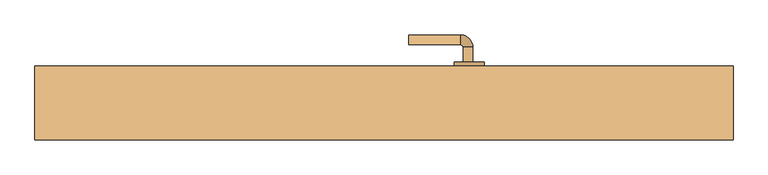
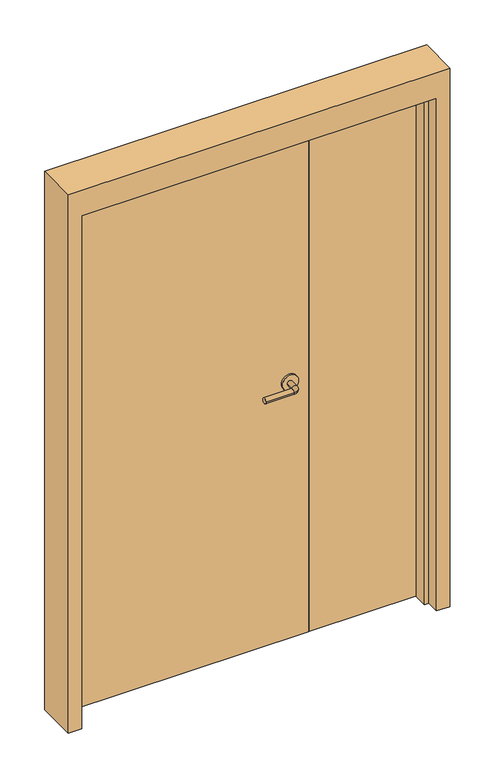
"""IFC4 building model written with IfcOpenShell, lengths in millimetres: door geometry, Дверь-Маятниковая-С полотнами разной ширины-Щитовая : 1410 x 2100 мм."""

import ifcopenshell
import ifcopenshell.guid

model = None  # the IFC model being written
_history = None  # IfcOwnerHistory: only IFC2X3 demands one
_inside = {}  # id of a spatial element -> (the spatial element, [elements in it])
_under = {}  # id of a project, library or spatial element -> (it, [spatial elements below it])
_declared = {}  # id of a project -> (the project, [libraries it declares])
_typed = {}  # id of a type object -> (the type object, [elements of that type])
_made_of = {}  # id of a material, layer set ... -> (it, [elements and type objects made of it])


def new_model(schema):
    """Start an empty IFC model of exactly this schema.

    Asked for "IFC4X3", IfcOpenShell would pick the latest addendum, in which some entities
    have other attributes; the version numbers below select the first issue.
    IFC2X3 requires an IfcOwnerHistory on every rooted entity: one is made here for all.
    """
    global model, _history
    if schema == "IFC4X3":
        model = ifcopenshell.file(schema_version=(4, 3, 0, 0))
    else:
        model = ifcopenshell.file(schema=schema)
    _inside.clear()
    _under.clear()
    _declared.clear()
    _typed.clear()
    _made_of.clear()
    _history = None
    if model.schema == "IFC2X3":
        org = make("IfcOrganization", Name="unknown")
        user = make(
            "IfcPersonAndOrganization",
            ThePerson=make("IfcPerson", FamilyName="unknown"),
            TheOrganization=org,
        )
        app = make(
            "IfcApplication",
            ApplicationDeveloper=org,
            Version="unknown",
            ApplicationFullName="unknown",
            ApplicationIdentifier="unknown",
        )
        _history = make(
            "IfcOwnerHistory",
            OwningUser=user,
            OwningApplication=app,
            ChangeAction="ADDED",
            CreationDate=0,
        )
    return model


def make(cls, **values):
    """One entity of the class cls with the attributes given. An attribute that is None is left unset."""
    return model.create_entity(
        cls, **{name: value for name, value in values.items() if value is not None}
    )


def rooted(cls, **values):
    """An entity with a GlobalId (a new one), such as an element, a storey or a relation."""
    return make(cls, GlobalId=ifcopenshell.guid.new(), OwnerHistory=_history, **values)


def si_unit(unit_type, name, prefix=None):
    """IfcSIUnit, for example si_unit("LENGTHUNIT", "METRE", prefix="MILLI")."""
    return make("IfcSIUnit", UnitType=unit_type, Prefix=prefix, Name=name)


def assignment(units):
    """IfcUnitAssignment: the units of a project."""
    return None if units is None else make("IfcUnitAssignment", Units=units)


def point(xyz):
    """IfcCartesianPoint."""
    return None if xyz is None else make("IfcCartesianPoint", Coordinates=xyz)


def direction(xyz):
    """IfcDirection."""
    return None if xyz is None else make("IfcDirection", DirectionRatios=xyz)


def frame(location, z_axis=None, x_axis=None):
    """IfcAxis2Placement3D, a coordinate frame: its origin and axes. An axis left out is left unset."""
    return make(
        "IfcAxis2Placement3D",
        Location=point(location),
        Axis=direction(z_axis),
        RefDirection=direction(x_axis),
    )


def frame_2d(location, x_axis=None):
    """IfcAxis2Placement2D, a coordinate frame in the plane: its origin and x axis."""
    return make(
        "IfcAxis2Placement2D", Location=point(location), RefDirection=direction(x_axis)
    )


def origin():
    """The frame at (0, 0, 0) with its axes left unset."""
    return frame((0.0, 0.0, 0.0))


def origin_with_axes():
    """The frame at (0, 0, 0) with the z axis (0, 0, 1) and the x axis (1, 0, 0) written out."""
    return frame((0.0, 0.0, 0.0), z_axis=(0.0, 0.0, 1.0), x_axis=(1.0, 0.0, 0.0))


def place(relative_to, where):
    """IfcLocalPlacement: puts the frame where relative to a parent placement (None: the world)."""
    return make(
        "IfcLocalPlacement", PlacementRelTo=relative_to, RelativePlacement=where
    )


def context(
    kind, dimensions, precision=None, world=None, true_north=None, identifier=None
):
    """IfcGeometricRepresentationContext, for example the 3D "Model" context."""
    return make(
        "IfcGeometricRepresentationContext",
        ContextIdentifier=identifier,
        ContextType=kind,
        CoordinateSpaceDimension=dimensions,
        Precision=precision,
        WorldCoordinateSystem=world,
        TrueNorth=true_north,
    )


def project(units=None, contexts=None):
    """IfcProject with its units and contexts."""
    return rooted(
        "IfcProject",
        Name="project",
        RepresentationContexts=contexts,
        UnitsInContext=assignment(units),
    )


def spatial(cls, under=None, at=None, **own):
    """A site, building, storey or space (cls), placed at a placement, below another one or the project."""
    s = rooted(cls, ObjectPlacement=at, **own)
    if under is not None:
        _under.setdefault(under.id(), (under, []))[1].append(s)
    return s


def polyline(points):
    """IfcPolyline through the points."""
    return make("IfcPolyline", Points=[point(p) for p in points])


def circle_curve(where, radius):
    """IfcCircle in the frame where."""
    return make("IfcCircle", Position=where, Radius=radius)


def ellipse_curve(where, semi_axis1, semi_axis2):
    """IfcEllipse in the frame where."""
    return make(
        "IfcEllipse", Position=where, SemiAxis1=semi_axis1, SemiAxis2=semi_axis2
    )


def trimmed(basis, trim1, trim2, sense, master):
    """IfcTrimmedCurve: the piece of a basis curve between two trims."""
    return make(
        "IfcTrimmedCurve",
        BasisCurve=basis,
        Trim1=trim1,
        Trim2=trim2,
        SenseAgreement=sense,
        MasterRepresentation=master,
    )


def segment(curve, same_sense, transition):
    """IfcCompositeCurveSegment."""
    return make(
        "IfcCompositeCurveSegment",
        Transition=transition,
        SameSense=same_sense,
        ParentCurve=curve,
    )


def composite_curve(segments, self_intersect=None):
    """IfcCompositeCurve: segments joined end to end."""
    return make("IfcCompositeCurve", Segments=segments, SelfIntersect=self_intersect)


def outline(outer, holes=None, kind="AREA"):
    """IfcArbitraryClosedProfileDef: a profile drawn as a closed curve; with holes, ...WithVoids."""
    if holes is None:
        return make("IfcArbitraryClosedProfileDef", ProfileType=kind, OuterCurve=outer)
    return make(
        "IfcArbitraryProfileDefWithVoids",
        ProfileType=kind,
        OuterCurve=outer,
        InnerCurves=holes,
    )


def extrude(swept, where, along, depth):
    """IfcExtrudedAreaSolid: the profile swept, set in the frame where, extruded along a direction by depth."""
    return make(
        "IfcExtrudedAreaSolid",
        SweptArea=swept,
        Position=where,
        ExtrudedDirection=direction(along),
        Depth=depth,
    )


def faces_of(points, faces, orient=None, outer=None):
    """IfcFace entities. A face is a list of loops; a loop is a list of indices into points, from 0.

    orient and outer hold one flag for each loop. By default every Orientation is true, the
    first loop of a face is its IfcFaceOuterBound and the others are IfcFaceBound.
    """
    made = []
    for i, loops in enumerate(faces):
        bounds = []
        for j, loop in enumerate(loops):
            is_outer = j == 0 if outer is None else outer[i][j]
            bounds.append(
                make(
                    "IfcFaceOuterBound" if is_outer else "IfcFaceBound",
                    Bound=make("IfcPolyLoop", Polygon=[points[k] for k in loop]),
                    Orientation=True if orient is None else orient[i][j],
                )
            )
        made.append(make("IfcFace", Bounds=bounds))
    return made


def faceted_brep(points, faces, orient=None, outer=None, voids=None):
    """IfcFacetedBrep: a solid bounded by flat faces; with voids (closed shells), ...WithVoids."""
    shared = [point(p) for p in points]
    hull = make("IfcClosedShell", CfsFaces=faces_of(shared, faces, orient, outer))
    if voids is None:
        return make("IfcFacetedBrep", Outer=hull)
    return make(
        "IfcFacetedBrepWithVoids",
        Outer=hull,
        Voids=[
            make(cls, CfsFaces=faces_of(shared, fs, o, b)) for cls, fs, o, b in voids
        ],
    )


def shape(context_of_items, identifier, shape_type, items):
    """IfcShapeRepresentation: the items that make up one representation, for example the "Body"."""
    return make(
        "IfcShapeRepresentation",
        ContextOfItems=context_of_items,
        RepresentationIdentifier=identifier,
        RepresentationType=shape_type,
        Items=items,
    )


def source(mapping_origin, context_of_items, identifier, shape_type, items):
    """IfcRepresentationMap: a shape defined once, which mapped items show again and again."""
    return make(
        "IfcRepresentationMap",
        MappingOrigin=mapping_origin,
        MappedRepresentation=shape(context_of_items, identifier, shape_type, items),
    )


def transform(
    local_origin,
    x_axis=None,
    y_axis=None,
    z_axis=None,
    scale=None,
    scale2=None,
    scale3=None,
    uniform=True,
):
    """IfcCartesianTransformationOperator3D, or its non-uniform kind. x_axis, y_axis, z_axis: its Axis1, 2, 3."""
    if uniform:
        return make(
            "IfcCartesianTransformationOperator3D",
            Axis1=direction(x_axis),
            Axis2=direction(y_axis),
            LocalOrigin=point(local_origin),
            Scale=scale,
            Axis3=direction(z_axis),
        )
    return make(
        "IfcCartesianTransformationOperator3DnonUniform",
        Axis1=direction(x_axis),
        Axis2=direction(y_axis),
        LocalOrigin=point(local_origin),
        Scale=scale,
        Axis3=direction(z_axis),
        Scale2=scale2,
        Scale3=scale3,
    )


def mapped(mapping_source, mapping_target):
    """IfcMappedItem: shows the shape of a source again, moved by a transform."""
    return make(
        "IfcMappedItem", MappingSource=mapping_source, MappingTarget=mapping_target
    )


def made_of(thing, what):
    """Note that an element or type object is made of a material, layer set ...; save() writes the relation."""
    if what is not None:
        _made_of.setdefault(what.id(), (what, []))[1].append(thing)
    return thing


def element(
    cls,
    number,
    at=None,
    inside=None,
    cuts=None,
    type_object=None,
    material=None,
    context=None,
    identifier="Body",
    shape_type=None,
    held_by="IfcProductDefinitionShape",
    body=None,
    shapes=None,
    **own,
):
    """One element of the class cls, such as IfcWall. Its Tag is "e" and its number.

    at: its placement. inside: the storey or other place that contains it. cuts: it is an
    opening in that element (IfcRelVoidsElement). A single representation is given by context,
    identifier, shape_type and body (its items); several are given by shapes. held_by: the class
    of the entity that holds the representations. save() writes the other relations.
    """
    e = rooted(cls, Tag="e%d" % number, ObjectPlacement=at, **own)
    if body is not None:
        shapes = [shape(context, identifier, shape_type, body)]
    if shapes is not None:
        e.Representation = make(held_by, Representations=shapes)
    if inside is not None:
        _inside.setdefault(inside.id(), (inside, []))[1].append(e)
    if cuts is not None:
        rooted(
            "IfcRelVoidsElement", RelatingBuildingElement=cuts, RelatedOpeningElement=e
        )
    if type_object is not None:
        _typed.setdefault(type_object.id(), (type_object, []))[1].append(e)
    return made_of(e, material)


def aggregate(whole, parts):
    """IfcRelAggregates: a whole, such as a stair, and the parts it consists of."""
    return rooted("IfcRelAggregates", RelatingObject=whole, RelatedObjects=parts)


def save(model, path):
    """Write the relations noted so far, then the file.

    IfcRelAggregates (storeys below a building ...), IfcRelContainedInSpatialStructure (elements
    in a storey), IfcRelDefinesByType, IfcRelAssociatesMaterial and IfcRelDeclares: one each for
    every whole, place, type object, material and project.
    """
    for whole, parts in _under.values():
        aggregate(whole, parts)
    for where, things in _inside.values():
        rooted(
            "IfcRelContainedInSpatialStructure",
            RelatedElements=things,
            RelatingStructure=where,
        )
    for kind, things in _typed.values():
        rooted("IfcRelDefinesByType", RelatedObjects=things, RelatingType=kind)
    for what, things in _made_of.values():
        rooted("IfcRelAssociatesMaterial", RelatedObjects=things, RelatingMaterial=what)
    for by, libraries in _declared.values():
        rooted("IfcRelDeclares", RelatingContext=by, RelatedDefinitions=libraries)
    model.write(path)


def plane_surface(at):
    """IfcPlane: the flat surface through the origin of the frame at, square to its z axis."""
    return make("IfcPlane", Position=at)


def cylinder_surface(at, radius):
    """IfcCylindricalSurface: all points at the distance radius from the z axis of the frame at."""
    return make("IfcCylindricalSurface", Position=at, Radius=radius)


def revolved_surface(curve, axis_point, axis_direction):
    """IfcSurfaceOfRevolution: the curve turned about the line through axis_point along axis_direction."""
    return make(
        "IfcSurfaceOfRevolution",
        SweptCurve=make("IfcArbitraryOpenProfileDef", ProfileType="CURVE", Curve=curve),
        AxisPosition=make("IfcAxis1Placement", Location=point(axis_point), Axis=direction(axis_direction)),
    )


def advanced_brep(points, edges, surfaces, faces):
    """IfcAdvancedBrep: a solid bounded by faces that lie on surfaces and meet in shared edges.

    An edge is (start, end): straight between two places in points (the first is 0);
    or (start, end, curve); or (start, end, curve, False) where it runs against its curve.
    A face is (place in surfaces, loops), or (place, loops, False) where it looks against
    its surface's normal. A loop lists edges by number (the first is 1), with a minus sign
    where the edge is run from its end to its start. The first loop is the outer one.
    """
    corners = [point(p) for p in points]
    vertices = [make("IfcVertexPoint", VertexGeometry=c) for c in corners]
    made = []
    for start, end, *more in edges:
        made.append(
            make(
                "IfcEdgeCurve",
                EdgeStart=vertices[start],
                EdgeEnd=vertices[end],
                EdgeGeometry=more[0] if more else make("IfcPolyline", Points=[corners[start], corners[end]]),
                SameSense=more[1] if len(more) > 1 else True,
            )
        )
    hull = []
    for where, loops, *sense in faces:
        bounds = []
        for j, loop in enumerate(loops):
            ring = [make("IfcOrientedEdge", EdgeElement=made[abs(k) - 1], Orientation=k > 0) for k in loop]
            bounds.append(
                make(
                    "IfcFaceOuterBound" if j == 0 else "IfcFaceBound",
                    Bound=make("IfcEdgeLoop", EdgeList=ring),
                    Orientation=True,
                )
            )
        hull.append(make("IfcAdvancedFace", Bounds=bounds, FaceSurface=surfaces[where], SameSense=sense[0] if sense else True))
    return make("IfcAdvancedBrep", Outer=make("IfcClosedShell", CfsFaces=hull))


def door_5009f339(model_context):
    return source(origin(), model_context, "Body", "SolidModel", [
        advanced_brep(
        [(179.59375, 118.35, 1000.0), (159.59375, 118.35, 1000.0), (179.59375, 88.35, 1000.0), (159.59375, 88.35, 1000.0), (154.59375, 83.35, 1000.0), (154.59375, 63.35, 1000.0), (49.59375, 63.35, 1000.0), (49.59375, 83.35, 1000.0)],
        [
            (0, 1, circle_curve(frame((169.59375, 118.35, 1000.0), z_axis=(0.0, 1.0, 0.0), x_axis=(-1.0, 0.0, 0.0)), 10.0)),
            (1, 0, circle_curve(frame((169.59375, 118.35, 1000.0), z_axis=(0.0, 1.0, 0.0), x_axis=(-1.0, 0.0, 0.0)), 10.0)),
            (0, 2),
            (2, 3, circle_curve(frame((169.59375, 88.35, 1000.0), z_axis=(0.0, 1.0, 0.0), x_axis=(-1.0, 0.0, 0.0)), 10.0)),
            (3, 1),
            (3, 2, circle_curve(frame((169.59375, 88.35, 1000.0), z_axis=(0.0, 1.0, 0.0), x_axis=(-1.0, 0.0, 0.0)), 10.0)),
            (4, 3, circle_curve(frame((154.59375, 88.35, 1000.0), z_axis=(0.0, 0.0, 1.0), x_axis=(1.0, 0.0, 0.0)), 5.0)),
            (2, 5, circle_curve(frame((154.59375, 88.35, 1000.0), z_axis=(0.0, 0.0, -1.0), x_axis=(1.0, 0.0, 0.0)), 25.0)),
            (5, 4, circle_curve(frame((154.59375, 73.35, 1000.0), z_axis=(1.0, 0.0, 0.0), x_axis=(0.0, 1.0, 0.0)), 10.0)),
            (4, 5, circle_curve(frame((154.59375, 73.35, 1000.0), z_axis=(1.0, 0.0, 0.0), x_axis=(0.0, 1.0, 0.0)), 10.0)),
            (6, 7, circle_curve(frame((49.59375, 73.35, 1000.0), z_axis=(-1.0, 0.0, 0.0), x_axis=(0.0, 1.0, 0.0)), 10.0)),
            (7, 6, circle_curve(frame((49.59375, 73.35, 1000.0), z_axis=(-1.0, 0.0, 0.0), x_axis=(0.0, 1.0, 0.0)), 10.0)),
            (5, 6),
            (7, 4),
        ],
        [
            plane_surface(frame((169.59375, 118.35, 1000.0), z_axis=(0.0, 1.0, 0.0), x_axis=(0.0, 0.0, 1.0))),
            cylinder_surface(frame((169.59375, 118.35, 1000.0), z_axis=(0.0, 1.0, 0.0), x_axis=(-1.0, 0.0, 0.0)), 10.0),
            revolved_surface(trimmed(ellipse_curve(frame((169.59375, 88.35, 1000.0), z_axis=(0.0, 1.0, 0.0), x_axis=(-1.0, 0.0, 0.0)), 10.0, 10.0), [point((179.59375, 88.35, 1000.0))], [point((159.59375, 88.35, 1000.0))], True, "CARTESIAN"), (154.59375, 88.35, 1000.0), (0.0, 0.0, -1.0)),
            revolved_surface(trimmed(ellipse_curve(frame((169.59375, 88.35, 1000.0), z_axis=(0.0, 1.0, 0.0), x_axis=(-1.0, 0.0, 0.0)), 10.0, 10.0), [point((159.59375, 88.35, 1000.0))], [point((179.59375, 88.35, 1000.0))], True, "CARTESIAN"), (154.59375, 88.35, 1000.0), (0.0, 0.0, -1.0)),
            plane_surface(frame((49.59375, 73.35, 1000.0), z_axis=(-1.0, 0.0, 0.0), x_axis=(0.0, 0.0, 1.0))),
            cylinder_surface(frame((154.59375, 73.35, 1000.0), z_axis=(1.0, 0.0, 0.0), x_axis=(0.0, 1.0, 0.0)), 10.0),
        ],
        [
            (0, [[1, 2]]),
            (1, [[-1, 3, 4, 5]]),
            (1, [[-2, -5, 6, -3]]),
            (2, [[7, -4, 8, 9]]),
            (3, [[-8, -6, -7, 10]]),
            (4, [[11, 12]]),
            (5, [[-9, 13, -12, 14]]),
            (5, [[-10, -14, -11, -13]]),
        ],
    ),
        extrude(outline(composite_curve([segment(trimmed(circle_curve(frame_2d((1000.0, 172.09375)), 30.0), [point((1000.0, 202.09375))], [point((1000.0, 142.09375))], False, "CARTESIAN"), True, "CONTINUOUS"), segment(trimmed(circle_curve(frame_2d((1000.0, 172.09375)), 30.0), [point((1000.0, 142.09375))], [point((1000.0, 202.09375))], False, "CARTESIAN"), True, "CONTINUOUS")], self_intersect=False)), frame((0.0, 118.35, 0.0), z_axis=(0.0, 1.0, 0.0), x_axis=(0.0, 0.0, 1.0)), (0.0, 0.0, 1.0), 8.0),
        advanced_brep(
        [(179.59375, 179.35, 1000.0), (159.59375, 179.35, 1000.0), (159.59375, 209.35, 1000.0), (179.59375, 209.35, 1000.0), (154.59375, 214.35, 1000.0), (154.59375, 234.35, 1000.0), (49.59375, 234.35, 1000.0), (49.59375, 214.35, 1000.0)],
        [
            (0, 1, circle_curve(frame((169.59375, 179.35, 1000.0), z_axis=(0.0, -1.0, 0.0), x_axis=(-1.0, 0.0, 0.0)), 10.0)),
            (1, 0, circle_curve(frame((169.59375, 179.35, 1000.0), z_axis=(0.0, -1.0, 0.0), x_axis=(-1.0, 0.0, 0.0)), 10.0)),
            (1, 2),
            (2, 3, circle_curve(frame((169.59375, 209.35, 1000.0), z_axis=(0.0, -1.0, 0.0), x_axis=(-1.0, 0.0, 0.0)), 10.0)),
            (3, 0),
            (3, 2, circle_curve(frame((169.59375, 209.35, 1000.0), z_axis=(0.0, -1.0, 0.0), x_axis=(-1.0, 0.0, 0.0)), 10.0)),
            (4, 5, circle_curve(frame((154.59375, 224.35, 1000.0), z_axis=(1.0, 0.0, 0.0), x_axis=(0.0, -1.0, 0.0)), 10.0)),
            (5, 3, circle_curve(frame((154.59375, 209.35, 1000.0), z_axis=(0.0, 0.0, -1.0), x_axis=(1.0, 0.0, 0.0)), 25.0)),
            (2, 4, circle_curve(frame((154.59375, 209.35, 1000.0), z_axis=(0.0, 0.0, 1.0), x_axis=(1.0, 0.0, 0.0)), 5.0)),
            (5, 4, circle_curve(frame((154.59375, 224.35, 1000.0), z_axis=(1.0, 0.0, 0.0), x_axis=(0.0, -1.0, 0.0)), 10.0)),
            (6, 7, circle_curve(frame((49.59375, 224.35, 1000.0), z_axis=(-1.0, 0.0, 0.0), x_axis=(0.0, -1.0, 0.0)), 10.0)),
            (7, 6, circle_curve(frame((49.59375, 224.35, 1000.0), z_axis=(-1.0, 0.0, 0.0), x_axis=(0.0, -1.0, 0.0)), 10.0)),
            (4, 7),
            (6, 5),
        ],
        [
            plane_surface(frame((169.59375, 179.35, 1000.0), z_axis=(0.0, -1.0, 0.0), x_axis=(0.0, 0.0, 1.0))),
            cylinder_surface(frame((169.59375, 179.35, 1000.0), z_axis=(0.0, -1.0, 0.0), x_axis=(-1.0, 0.0, 0.0)), 10.0),
            revolved_surface(trimmed(ellipse_curve(frame((169.59375, 209.35, 1000.0), z_axis=(0.0, 1.0, 0.0), x_axis=(-1.0, 0.0, 0.0)), 10.0, 10.0), [point((179.59375, 209.35, 1000.0))], [point((159.59375, 209.35, 1000.0))], True, "CARTESIAN"), (154.59375, 209.35, 1000.0), (0.0, 0.0, -1.0)),
            revolved_surface(trimmed(ellipse_curve(frame((169.59375, 209.35, 1000.0), z_axis=(0.0, 1.0, 0.0), x_axis=(-1.0, 0.0, 0.0)), 10.0, 10.0), [point((159.59375, 209.35, 1000.0))], [point((179.59375, 209.35, 1000.0))], True, "CARTESIAN"), (154.59375, 209.35, 1000.0), (0.0, 0.0, -1.0)),
            plane_surface(frame((49.59375, 224.35, 1000.0), z_axis=(-1.0, 0.0, 0.0), x_axis=(0.0, 0.0, 1.0))),
            cylinder_surface(frame((154.59375, 224.35, 1000.0), z_axis=(1.0, 0.0, 0.0), x_axis=(0.0, -1.0, 0.0)), 10.0),
        ],
        [
            (0, [[1, 2]]),
            (1, [[3, 4, 5, -2]]),
            (1, [[-5, 6, -3, -1]]),
            (2, [[7, 8, -4, 9]]),
            (3, [[10, -9, -6, -8]]),
            (4, [[11, 12]]),
            (5, [[13, -11, 14, -7]]),
            (5, [[-14, -12, -13, -10]]),
        ],
    ),
        extrude(outline(composite_curve([segment(trimmed(circle_curve(frame_2d((1000.0, 172.09375)), 30.0), [point((1000.0, 202.09375))], [point((1000.0, 142.09375))], False, "CARTESIAN"), True, "CONTINUOUS"), segment(trimmed(circle_curve(frame_2d((1000.0, 172.09375)), 30.0), [point((1000.0, 142.09375))], [point((1000.0, 202.09375))], False, "CARTESIAN"), True, "CONTINUOUS")], self_intersect=False)), frame((0.0, 171.35, 0.0), z_axis=(0.0, 1.0, 0.0), x_axis=(0.0, 0.0, 1.0)), (0.0, 0.0, 1.0), 8.0),
        extrude(outline(polyline([(655.0, 126.35), (246.6, 126.35), (246.6, 171.35), (655.0, 171.35), (655.0, 126.35)])), origin_with_axes(), (0.0, 0.0, 1.0), 2000.0),
        faceted_brep([(655.0, 121.5875, 0.0), (655.0, 171.35, 0.0), (705.0, 171.35, 0.0), (705.0, 21.35, 0.0), (655.0, 21.35, 0.0), (655.0, 70.5625, 0.0), (639.125, 70.5625, 0.0), (639.125, 121.5875, 0.0), (655.0, 121.5875, 2000.0), (655.0, 171.35, 2000.0), (-655.0, 171.35, 2000.0), (-655.0, 171.35, 0.0), (-705.0, 171.35, 0.0), (-705.0, 171.35, 2100.0), (705.0, 171.35, 2100.0), (705.0, 21.35, 2100.0), (-705.0, 21.35, 2100.0), (-705.0, 21.35, 0.0), (-655.0, 21.35, 0.0), (-655.0, 21.35, 2000.0), (655.0, 21.35, 2000.0), (655.0, 70.5625, 2000.0), (-655.0, 70.5625, 2000.0), (-655.0, 70.5625, 0.0), (-639.125, 70.5625, 0.0), (-639.125, 70.5625, 1984.125), (639.125, 70.5625, 1984.125), (639.125, 121.5875, 1984.125), (-639.125, 121.5875, 1984.125), (-639.125, 121.5875, 0.0), (-655.0, 121.5875, 0.0), (-655.0, 121.5875, 2000.0)], [[[0, 1, 2, 3, 4, 5, 6, 7]], [[1, 0, 8, 9]], [[2, 1, 9, 10, 11, 12, 13, 14]], [[3, 2, 14, 15]], [[4, 3, 15, 16, 17, 18, 19, 20]], [[5, 4, 20, 21]], [[6, 5, 21, 22, 23, 24, 25, 26]], [[7, 6, 26, 27]], [[0, 7, 27, 28, 29, 30, 31, 8]], [[9, 8, 31, 10]], [[20, 19, 22, 21]], [[26, 25, 28, 27]], [[12, 11, 30, 29, 24, 23, 18, 17]], [[11, 10, 31, 30]], [[13, 12, 17, 16]], [[19, 18, 23, 22]], [[25, 24, 29, 28]], [[15, 14, 13, 16]]]),
        extrude(outline(polyline([(243.4, 126.35), (-655.0, 126.35), (-655.0, 171.35), (243.4, 171.35), (243.4, 126.35)])), origin_with_axes(), (0.0, 0.0, 1.0), 2000.0),
    ])


if __name__ == "__main__":
    model = new_model("IFC4")
    model_context = context("Model", 3, world=origin())
    ifc_project = project(units=[si_unit("LENGTHUNIT", "METRE", prefix="MILLI")], contexts=[model_context])
    site = spatial("IfcSite", under=ifc_project)
    building = spatial("IfcBuilding", under=site)
    placement = place(None, origin())
    door_shape = door_5009f339(model_context)
    element("IfcDoor", 1, ObjectType="Дверь-Маятниковая-С полотнами разной ширины-Щитовая : 1410 x 2100 мм", at=placement, inside=building, context=model_context, shape_type="MappedRepresentation", body=[
        mapped(door_shape, transform((0.0, 0.0, 0.0), x_axis=(1.0, 0.0, 0.0), y_axis=(0.0, 1.0, 0.0), z_axis=(0.0, 0.0, 1.0))),
    ])
    save(model, "model.ifc")

# Revit data of these elements
# Type "Дверь-Маятниковая-С полотнами разной ширины-Щитовая : 1410 x 2100 мм"
#   Type Mark = "155"
#   Assembly Code = "C1020300"
#   Analytic Construction = "Деревянный"
#   Ширина большой панели = 900 mm
#   W = 410 mm
#   Thickness = 45 mm
#   Thermal Resistance (R) = 0.455703 (m²·K)/W
#   Угол поворота [instance default] = 90°
#   Высота планки = 1000 mm
#   Rough Width [instance default] = 1410 mm
#   Rough Height [instance default] = 2100 mm
#   Высота проема в кирпичном каркасе [instance default] = 100 mm
#   Ширина проема в кирпичном каркасе [instance default] = 100 mm
#   Расчет вставки [instance default] = 105 mm
#   Кирпичная вставка [instance default] = 25 mm
#   Height = 2000 mm
#   Width = 1310 mm
#   Heat Transfer Coefficient (U) = 2.19465 W/(m²·K)
#   Глубина кирпичного каркаса = 150 mm
#   Кирпичный каркас [instance default] = yes
#   Каркас стены сухой кладки [instance default] = no
#   Материал панели = Древесина - Береза
#   Материал каркаса = Металл - Окрашенный - Серый 2
#   Материал дверной ручки = Алюминий
#   Visual Light Transmittance = 0
#   Solar Heat Gain Coefficient = 0
#   Wall Closure = (empty or 0)
#   Function = (empty or 0)
# Element 1 (IfcDoor, "Дверь-Маятниковая-С полотнами разной ширины-Щитовая : 1410 x 2100 мм")
#   Materials on its faces: "Алюминий", "Металл - Окрашенный - Серый 2", "Древесина - Береза"
# Materials
#   "Древесина - Береза": class "Древесина", colour RGB 166 116 52, transparency 0, Cost = 0
#   "Металл - Окрашенный - Серый 2": class "Краска", colour RGB 104 104 104, transparency 0, Cost = 0
#   "Алюминий": class "Металл", colour RGB 247 247 247, transparency 0
